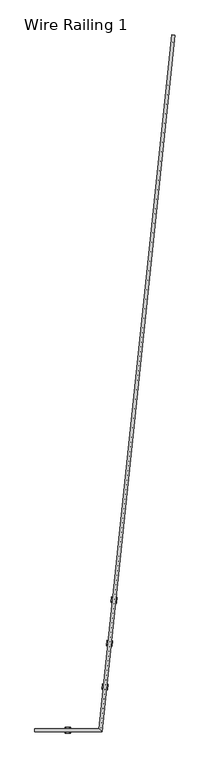
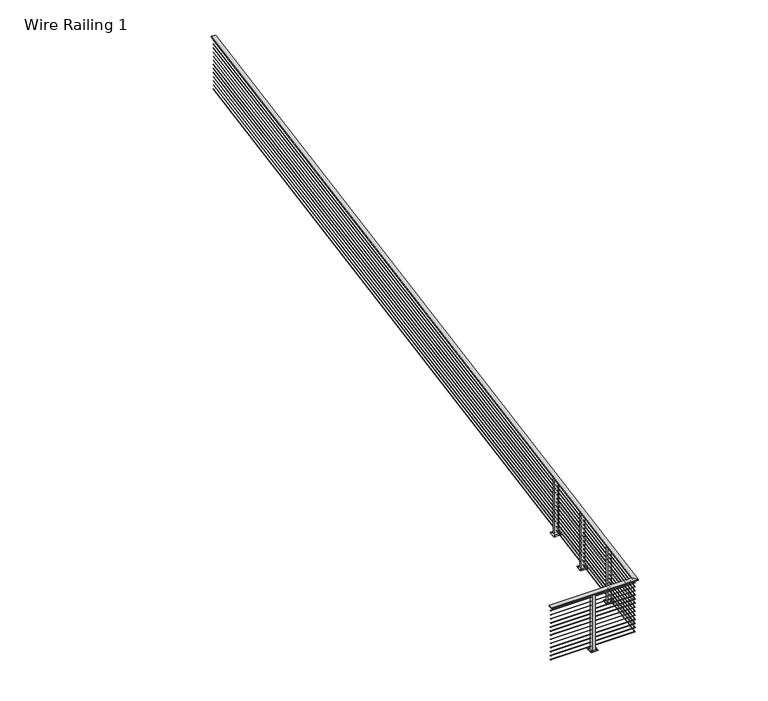
"""IFC4 building model written with IfcOpenShell, lengths in millimetres: railing geometry, Wire Railing 1."""

from ifc_helpers import new_model, si_unit, point, frame, frame_2d, origin, place, context, project, spatial, polyline, circle_curve, ellipse_curve, trimmed, segment, composite_curve, outline, extrude, faceted_brep, source, transform, mapped, element, save
from ifc_brep_helpers import plane_surface, cylinder_surface, advanced_brep


def wire_railing_1_8b9fc924(model_context):
    return source(origin(), model_context, "Body", "SolidModel", [
        faceted_brep([(32234.7381966, 25546.7031612, 267462.0), (32234.7381966, 25622.9031612, 267462.0), (32234.7381966, 25622.9031612, 267442.95), (32234.7381966, 25546.7031612, 267442.95), (33761.2935907, 25546.7031612, 267462.0), (33692.6828025, 25622.9031612, 267462.0), (33692.6828025, 25622.9031612, 267442.95), (33761.2935907, 25546.7031612, 267442.95), (35422.3408934, 41350.5125752, 267462.0), (35422.3408934, 41350.5125752, 267442.95), (35346.558325, 41358.4776441, 267442.95), (35346.558325, 41358.4776441, 267462.0)], [[[0, 1, 2, 3]], [[4, 5, 1, 0]], [[5, 6, 2, 1]], [[6, 7, 3, 2]], [[7, 4, 0, 3]], [[8, 9, 10, 11]], [[9, 8, 4, 7]], [[10, 9, 7, 6]], [[11, 10, 6, 5]], [[8, 11, 5, 4]]]),
        advanced_brep(
        [(32234.7381966, 25587.1844112, 267383.41875), (32234.7381966, 25582.4219112, 267383.41875), (33724.8441095, 25587.1844112, 267383.41875), (33729.1322837, 25582.4219112, 267383.41875), (35382.081404, 41354.7440181, 267383.41875), (35386.8178145, 41354.2462013, 267383.41875)],
        [
            (0, 1, circle_curve(frame((32234.7381966, 25584.8031612, 267383.41875), z_axis=(-1.0, 0.0, 0.0), x_axis=(0.0, -1.0, 0.0)), 2.38125)),
            (1, 0, circle_curve(frame((32234.7381966, 25584.8031612, 267383.41875), z_axis=(-1.0, 0.0, 0.0), x_axis=(0.0, -1.0, 0.0)), 2.38125)),
            (2, 3, ellipse_curve(frame((33726.9881966, 25584.8031612, 267383.41875), z_axis=(-0.7431448254773928, -0.66913060635886, 0.0), x_axis=(0.6691306063588597, -0.7431448254773928, 0.0)), 3.2042879, 2.38125)),
            (3, 1),
            (0, 2),
            (3, 2, ellipse_curve(frame((33726.9881966, 25584.8031612, 267383.41875), z_axis=(-0.7431448254773928, -0.66913060635886, 0.0), x_axis=(0.6691306063588597, -0.7431448254773928, 0.0)), 3.2042879, 2.38125)),
            (4, 5, circle_curve(frame((35384.4496092, 41354.4951097, 267383.41875), z_axis=(0.10452846326764917, 0.9945218953682738, 0.0), x_axis=(0.9945218953682738, -0.10452846326764917, 0.0)), 2.38125)),
            (5, 4, circle_curve(frame((35384.4496092, 41354.4951097, 267383.41875), z_axis=(0.10452846326764917, 0.9945218953682738, 0.0), x_axis=(0.9945218953682738, -0.10452846326764917, 0.0)), 2.38125)),
            (4, 2),
            (3, 5),
        ],
        [
            plane_surface(frame((32234.7381966, 25584.8031612, 267385.8), z_axis=(-1.0, 0.0, 0.0), x_axis=(0.0, -1.0, 0.0))),
            cylinder_surface(frame((33726.9881966, 25584.8031612, 267383.41875), z_axis=(1.0, 0.0, 0.0), x_axis=(0.0, -1.0, 0.0)), 2.38125),
            plane_surface(frame((35384.4496092, 41354.4951097, 267385.8), z_axis=(0.10452846326764917, 0.9945218953682738, 0.0), x_axis=(0.9945218953682738, -0.10452846326764917, 0.0))),
            cylinder_surface(frame((35384.4496092, 41354.4951097, 267383.41875), z_axis=(0.10452846326764917, 0.9945218953682738, 0.0), x_axis=(0.9945218953682738, -0.10452846326764917, 0.0)), 2.38125),
        ],
        [
            (0, [[1, 2]]),
            (1, [[3, 4, -1, 5]]),
            (1, [[6, -5, -2, -4]]),
            (2, [[7, 8]]),
            (3, [[-7, 9, -6, 10]]),
            (3, [[-8, -10, -3, -9]]),
        ],
    ),
        advanced_brep(
        [(32234.7381966, 25587.1844112, 267307.21875), (32234.7381966, 25582.4219112, 267307.21875), (33724.8441095, 25587.1844112, 267307.21875), (33729.1322837, 25582.4219112, 267307.21875), (35382.081404, 41354.7440181, 267307.21875), (35386.8178145, 41354.2462013, 267307.21875)],
        [
            (0, 1, circle_curve(frame((32234.7381966, 25584.8031612, 267307.21875), z_axis=(-1.0, 0.0, 0.0), x_axis=(0.0, -1.0, 0.0)), 2.38125)),
            (1, 0, circle_curve(frame((32234.7381966, 25584.8031612, 267307.21875), z_axis=(-1.0, 0.0, 0.0), x_axis=(0.0, -1.0, 0.0)), 2.38125)),
            (2, 3, ellipse_curve(frame((33726.9881966, 25584.8031612, 267307.21875), z_axis=(-0.7431448254773928, -0.66913060635886, 0.0), x_axis=(0.6691306063588597, -0.7431448254773928, 0.0)), 3.2042879, 2.38125)),
            (3, 1),
            (0, 2),
            (3, 2, ellipse_curve(frame((33726.9881966, 25584.8031612, 267307.21875), z_axis=(-0.7431448254773928, -0.66913060635886, 0.0), x_axis=(0.6691306063588597, -0.7431448254773928, 0.0)), 3.2042879, 2.38125)),
            (4, 5, circle_curve(frame((35384.4496092, 41354.4951097, 267307.21875), z_axis=(0.10452846326764917, 0.9945218953682738, 0.0), x_axis=(0.9945218953682738, -0.10452846326764917, 0.0)), 2.38125)),
            (5, 4, circle_curve(frame((35384.4496092, 41354.4951097, 267307.21875), z_axis=(0.10452846326764917, 0.9945218953682738, 0.0), x_axis=(0.9945218953682738, -0.10452846326764917, 0.0)), 2.38125)),
            (4, 2),
            (3, 5),
        ],
        [
            plane_surface(frame((32234.7381966, 25584.8031612, 267309.6), z_axis=(-1.0, 0.0, 0.0), x_axis=(0.0, -1.0, 0.0))),
            cylinder_surface(frame((33726.9881966, 25584.8031612, 267307.21875), z_axis=(1.0, 0.0, 0.0), x_axis=(0.0, -1.0, 0.0)), 2.38125),
            plane_surface(frame((35384.4496092, 41354.4951097, 267309.6), z_axis=(0.10452846326764917, 0.9945218953682738, 0.0), x_axis=(0.9945218953682738, -0.10452846326764917, 0.0))),
            cylinder_surface(frame((35384.4496092, 41354.4951097, 267307.21875), z_axis=(0.10452846326764917, 0.9945218953682738, 0.0), x_axis=(0.9945218953682738, -0.10452846326764917, 0.0)), 2.38125),
        ],
        [
            (0, [[1, 2]]),
            (1, [[3, 4, -1, 5]]),
            (1, [[6, -5, -2, -4]]),
            (2, [[7, 8]]),
            (3, [[-7, 9, -6, 10]]),
            (3, [[-8, -10, -3, -9]]),
        ],
    ),
        advanced_brep(
        [(32234.7381966, 25587.1844112, 267231.01875), (32234.7381966, 25582.4219112, 267231.01875), (33724.8441095, 25587.1844112, 267231.01875), (33729.1322837, 25582.4219112, 267231.01875), (35382.081404, 41354.7440181, 267231.01875), (35386.8178145, 41354.2462013, 267231.01875)],
        [
            (0, 1, circle_curve(frame((32234.7381966, 25584.8031612, 267231.01875), z_axis=(-1.0, 0.0, 0.0), x_axis=(0.0, -1.0, 0.0)), 2.38125)),
            (1, 0, circle_curve(frame((32234.7381966, 25584.8031612, 267231.01875), z_axis=(-1.0, 0.0, 0.0), x_axis=(0.0, -1.0, 0.0)), 2.38125)),
            (2, 3, ellipse_curve(frame((33726.9881966, 25584.8031612, 267231.01875), z_axis=(-0.7431448254773928, -0.66913060635886, 0.0), x_axis=(0.6691306063588597, -0.7431448254773928, 0.0)), 3.2042879, 2.38125)),
            (3, 1),
            (0, 2),
            (3, 2, ellipse_curve(frame((33726.9881966, 25584.8031612, 267231.01875), z_axis=(-0.7431448254773928, -0.66913060635886, 0.0), x_axis=(0.6691306063588597, -0.7431448254773928, 0.0)), 3.2042879, 2.38125)),
            (4, 5, circle_curve(frame((35384.4496092, 41354.4951097, 267231.01875), z_axis=(0.10452846326764917, 0.9945218953682738, 0.0), x_axis=(0.9945218953682738, -0.10452846326764917, 0.0)), 2.38125)),
            (5, 4, circle_curve(frame((35384.4496092, 41354.4951097, 267231.01875), z_axis=(0.10452846326764917, 0.9945218953682738, 0.0), x_axis=(0.9945218953682738, -0.10452846326764917, 0.0)), 2.38125)),
            (4, 2),
            (3, 5),
        ],
        [
            plane_surface(frame((32234.7381966, 25584.8031612, 267233.4), z_axis=(-1.0, 0.0, 0.0), x_axis=(0.0, -1.0, 0.0))),
            cylinder_surface(frame((33726.9881966, 25584.8031612, 267231.01875), z_axis=(1.0, 0.0, 0.0), x_axis=(0.0, -1.0, 0.0)), 2.38125),
            plane_surface(frame((35384.4496092, 41354.4951097, 267233.4), z_axis=(0.10452846326764917, 0.9945218953682738, 0.0), x_axis=(0.9945218953682738, -0.10452846326764917, 0.0))),
            cylinder_surface(frame((35384.4496092, 41354.4951097, 267231.01875), z_axis=(0.10452846326764917, 0.9945218953682738, 0.0), x_axis=(0.9945218953682738, -0.10452846326764917, 0.0)), 2.38125),
        ],
        [
            (0, [[1, 2]]),
            (1, [[3, 4, -1, 5]]),
            (1, [[6, -5, -2, -4]]),
            (2, [[7, 8]]),
            (3, [[-7, 9, -6, 10]]),
            (3, [[-8, -10, -3, -9]]),
        ],
    ),
        advanced_brep(
        [(32234.7381966, 25587.1844112, 267154.81875), (32234.7381966, 25582.4219112, 267154.81875), (33724.8441095, 25587.1844112, 267154.81875), (33729.1322837, 25582.4219112, 267154.81875), (35382.081404, 41354.7440181, 267154.81875), (35386.8178145, 41354.2462013, 267154.81875)],
        [
            (0, 1, circle_curve(frame((32234.7381966, 25584.8031612, 267154.81875), z_axis=(-1.0, 0.0, 0.0), x_axis=(0.0, -1.0, 0.0)), 2.38125)),
            (1, 0, circle_curve(frame((32234.7381966, 25584.8031612, 267154.81875), z_axis=(-1.0, 0.0, 0.0), x_axis=(0.0, -1.0, 0.0)), 2.38125)),
            (2, 3, ellipse_curve(frame((33726.9881966, 25584.8031612, 267154.81875), z_axis=(-0.7431448254773928, -0.66913060635886, 0.0), x_axis=(0.6691306063588597, -0.7431448254773928, 0.0)), 3.2042879, 2.38125)),
            (3, 1),
            (0, 2),
            (3, 2, ellipse_curve(frame((33726.9881966, 25584.8031612, 267154.81875), z_axis=(-0.7431448254773928, -0.66913060635886, 0.0), x_axis=(0.6691306063588597, -0.7431448254773928, 0.0)), 3.2042879, 2.38125)),
            (4, 5, circle_curve(frame((35384.4496092, 41354.4951097, 267154.81875), z_axis=(0.10452846326764917, 0.9945218953682738, 0.0), x_axis=(0.9945218953682738, -0.10452846326764917, 0.0)), 2.38125)),
            (5, 4, circle_curve(frame((35384.4496092, 41354.4951097, 267154.81875), z_axis=(0.10452846326764917, 0.9945218953682738, 0.0), x_axis=(0.9945218953682738, -0.10452846326764917, 0.0)), 2.38125)),
            (4, 2),
            (3, 5),
        ],
        [
            plane_surface(frame((32234.7381966, 25584.8031612, 267157.2), z_axis=(-1.0, 0.0, 0.0), x_axis=(0.0, -1.0, 0.0))),
            cylinder_surface(frame((33726.9881966, 25584.8031612, 267154.81875), z_axis=(1.0, 0.0, 0.0), x_axis=(0.0, -1.0, 0.0)), 2.38125),
            plane_surface(frame((35384.4496092, 41354.4951097, 267157.2), z_axis=(0.10452846326764917, 0.9945218953682738, 0.0), x_axis=(0.9945218953682738, -0.10452846326764917, 0.0))),
            cylinder_surface(frame((35384.4496092, 41354.4951097, 267154.81875), z_axis=(0.10452846326764917, 0.9945218953682738, 0.0), x_axis=(0.9945218953682738, -0.10452846326764917, 0.0)), 2.38125),
        ],
        [
            (0, [[1, 2]]),
            (1, [[3, 4, -1, 5]]),
            (1, [[6, -5, -2, -4]]),
            (2, [[7, 8]]),
            (3, [[-7, 9, -6, 10]]),
            (3, [[-8, -10, -3, -9]]),
        ],
    ),
        advanced_brep(
        [(32234.7381966, 25587.1844112, 267078.61875), (32234.7381966, 25582.4219112, 267078.61875), (33724.8441095, 25587.1844112, 267078.61875), (33729.1322837, 25582.4219112, 267078.61875), (35382.081404, 41354.7440181, 267078.61875), (35386.8178145, 41354.2462013, 267078.61875)],
        [
            (0, 1, circle_curve(frame((32234.7381966, 25584.8031612, 267078.61875), z_axis=(-1.0, 0.0, 0.0), x_axis=(0.0, -1.0, 0.0)), 2.38125)),
            (1, 0, circle_curve(frame((32234.7381966, 25584.8031612, 267078.61875), z_axis=(-1.0, 0.0, 0.0), x_axis=(0.0, -1.0, 0.0)), 2.38125)),
            (2, 3, ellipse_curve(frame((33726.9881966, 25584.8031612, 267078.61875), z_axis=(-0.7431448254773928, -0.66913060635886, 0.0), x_axis=(0.6691306063588597, -0.7431448254773928, 0.0)), 3.2042879, 2.38125)),
            (3, 1),
            (0, 2),
            (3, 2, ellipse_curve(frame((33726.9881966, 25584.8031612, 267078.61875), z_axis=(-0.7431448254773928, -0.66913060635886, 0.0), x_axis=(0.6691306063588597, -0.7431448254773928, 0.0)), 3.2042879, 2.38125)),
            (4, 5, circle_curve(frame((35384.4496092, 41354.4951097, 267078.61875), z_axis=(0.10452846326764917, 0.9945218953682738, 0.0), x_axis=(0.9945218953682738, -0.10452846326764917, 0.0)), 2.38125)),
            (5, 4, circle_curve(frame((35384.4496092, 41354.4951097, 267078.61875), z_axis=(0.10452846326764917, 0.9945218953682738, 0.0), x_axis=(0.9945218953682738, -0.10452846326764917, 0.0)), 2.38125)),
            (4, 2),
            (3, 5),
        ],
        [
            plane_surface(frame((32234.7381966, 25584.8031612, 267081.0), z_axis=(-1.0, 0.0, 0.0), x_axis=(0.0, -1.0, 0.0))),
            cylinder_surface(frame((33726.9881966, 25584.8031612, 267078.61875), z_axis=(1.0, 0.0, 0.0), x_axis=(0.0, -1.0, 0.0)), 2.38125),
            plane_surface(frame((35384.4496092, 41354.4951097, 267081.0), z_axis=(0.10452846326764917, 0.9945218953682738, 0.0), x_axis=(0.9945218953682738, -0.10452846326764917, 0.0))),
            cylinder_surface(frame((35384.4496092, 41354.4951097, 267078.61875), z_axis=(0.10452846326764917, 0.9945218953682738, 0.0), x_axis=(0.9945218953682738, -0.10452846326764917, 0.0)), 2.38125),
        ],
        [
            (0, [[1, 2]]),
            (1, [[3, 4, -1, 5]]),
            (1, [[6, -5, -2, -4]]),
            (2, [[7, 8]]),
            (3, [[-7, 9, -6, 10]]),
            (3, [[-8, -10, -3, -9]]),
        ],
    ),
        advanced_brep(
        [(32234.7381966, 25587.1844112, 267002.41875), (32234.7381966, 25582.4219112, 267002.41875), (33724.8441095, 25587.1844112, 267002.41875), (33729.1322837, 25582.4219112, 267002.41875), (35382.081404, 41354.7440181, 267002.41875), (35386.8178145, 41354.2462013, 267002.41875)],
        [
            (0, 1, circle_curve(frame((32234.7381966, 25584.8031612, 267002.41875), z_axis=(-1.0, 0.0, 0.0), x_axis=(0.0, -1.0, 0.0)), 2.38125)),
            (1, 0, circle_curve(frame((32234.7381966, 25584.8031612, 267002.41875), z_axis=(-1.0, 0.0, 0.0), x_axis=(0.0, -1.0, 0.0)), 2.38125)),
            (2, 3, ellipse_curve(frame((33726.9881966, 25584.8031612, 267002.41875), z_axis=(-0.7431448254773928, -0.66913060635886, 0.0), x_axis=(0.6691306063588597, -0.7431448254773928, 0.0)), 3.2042879, 2.38125)),
            (3, 1),
            (0, 2),
            (3, 2, ellipse_curve(frame((33726.9881966, 25584.8031612, 267002.41875), z_axis=(-0.7431448254773928, -0.66913060635886, 0.0), x_axis=(0.6691306063588597, -0.7431448254773928, 0.0)), 3.2042879, 2.38125)),
            (4, 5, circle_curve(frame((35384.4496092, 41354.4951097, 267002.41875), z_axis=(0.10452846326764917, 0.9945218953682738, 0.0), x_axis=(0.9945218953682738, -0.10452846326764917, 0.0)), 2.38125)),
            (5, 4, circle_curve(frame((35384.4496092, 41354.4951097, 267002.41875), z_axis=(0.10452846326764917, 0.9945218953682738, 0.0), x_axis=(0.9945218953682738, -0.10452846326764917, 0.0)), 2.38125)),
            (4, 2),
            (3, 5),
        ],
        [
            plane_surface(frame((32234.7381966, 25584.8031612, 267004.8), z_axis=(-1.0, 0.0, 0.0), x_axis=(0.0, -1.0, 0.0))),
            cylinder_surface(frame((33726.9881966, 25584.8031612, 267002.41875), z_axis=(1.0, 0.0, 0.0), x_axis=(0.0, -1.0, 0.0)), 2.38125),
            plane_surface(frame((35384.4496092, 41354.4951097, 267004.8), z_axis=(0.10452846326764917, 0.9945218953682738, 0.0), x_axis=(0.9945218953682738, -0.10452846326764917, 0.0))),
            cylinder_surface(frame((35384.4496092, 41354.4951097, 267002.41875), z_axis=(0.10452846326764917, 0.9945218953682738, 0.0), x_axis=(0.9945218953682738, -0.10452846326764917, 0.0)), 2.38125),
        ],
        [
            (0, [[1, 2]]),
            (1, [[3, 4, -1, 5]]),
            (1, [[6, -5, -2, -4]]),
            (2, [[7, 8]]),
            (3, [[-7, 9, -6, 10]]),
            (3, [[-8, -10, -3, -9]]),
        ],
    ),
        advanced_brep(
        [(32234.7381966, 25587.1844112, 266926.21875), (32234.7381966, 25582.4219112, 266926.21875), (33724.8441095, 25587.1844112, 266926.21875), (33729.1322837, 25582.4219112, 266926.21875), (35382.081404, 41354.7440181, 266926.21875), (35386.8178145, 41354.2462013, 266926.21875)],
        [
            (0, 1, circle_curve(frame((32234.7381966, 25584.8031612, 266926.21875), z_axis=(-1.0, 0.0, 0.0), x_axis=(0.0, -1.0, 0.0)), 2.38125)),
            (1, 0, circle_curve(frame((32234.7381966, 25584.8031612, 266926.21875), z_axis=(-1.0, 0.0, 0.0), x_axis=(0.0, -1.0, 0.0)), 2.38125)),
            (2, 3, ellipse_curve(frame((33726.9881966, 25584.8031612, 266926.21875), z_axis=(-0.7431448254773928, -0.66913060635886, 0.0), x_axis=(0.6691306063588597, -0.7431448254773928, 0.0)), 3.2042879, 2.38125)),
            (3, 1),
            (0, 2),
            (3, 2, ellipse_curve(frame((33726.9881966, 25584.8031612, 266926.21875), z_axis=(-0.7431448254773928, -0.66913060635886, 0.0), x_axis=(0.6691306063588597, -0.7431448254773928, 0.0)), 3.2042879, 2.38125)),
            (4, 5, circle_curve(frame((35384.4496092, 41354.4951097, 266926.21875), z_axis=(0.10452846326764917, 0.9945218953682738, 0.0), x_axis=(0.9945218953682738, -0.10452846326764917, 0.0)), 2.38125)),
            (5, 4, circle_curve(frame((35384.4496092, 41354.4951097, 266926.21875), z_axis=(0.10452846326764917, 0.9945218953682738, 0.0), x_axis=(0.9945218953682738, -0.10452846326764917, 0.0)), 2.38125)),
            (4, 2),
            (3, 5),
        ],
        [
            plane_surface(frame((32234.7381966, 25584.8031612, 266928.6), z_axis=(-1.0, 0.0, 0.0), x_axis=(0.0, -1.0, 0.0))),
            cylinder_surface(frame((33726.9881966, 25584.8031612, 266926.21875), z_axis=(1.0, 0.0, 0.0), x_axis=(0.0, -1.0, 0.0)), 2.38125),
            plane_surface(frame((35384.4496092, 41354.4951097, 266928.6), z_axis=(0.10452846326764917, 0.9945218953682738, 0.0), x_axis=(0.9945218953682738, -0.10452846326764917, 0.0))),
            cylinder_surface(frame((35384.4496092, 41354.4951097, 266926.21875), z_axis=(0.10452846326764917, 0.9945218953682738, 0.0), x_axis=(0.9945218953682738, -0.10452846326764917, 0.0)), 2.38125),
        ],
        [
            (0, [[1, 2]]),
            (1, [[3, 4, -1, 5]]),
            (1, [[6, -5, -2, -4]]),
            (2, [[7, 8]]),
            (3, [[-7, 9, -6, 10]]),
            (3, [[-8, -10, -3, -9]]),
        ],
    ),
        advanced_brep(
        [(32234.7381966, 25587.1844112, 266850.01875), (32234.7381966, 25582.4219112, 266850.01875), (33724.8441095, 25587.1844112, 266850.01875), (33729.1322837, 25582.4219112, 266850.01875), (35382.081404, 41354.7440181, 266850.01875), (35386.8178145, 41354.2462013, 266850.01875)],
        [
            (0, 1, circle_curve(frame((32234.7381966, 25584.8031612, 266850.01875), z_axis=(-1.0, 0.0, 0.0), x_axis=(0.0, -1.0, 0.0)), 2.38125)),
            (1, 0, circle_curve(frame((32234.7381966, 25584.8031612, 266850.01875), z_axis=(-1.0, 0.0, 0.0), x_axis=(0.0, -1.0, 0.0)), 2.38125)),
            (2, 3, ellipse_curve(frame((33726.9881966, 25584.8031612, 266850.01875), z_axis=(-0.7431448254773928, -0.66913060635886, 0.0), x_axis=(0.6691306063588597, -0.7431448254773928, 0.0)), 3.2042879, 2.38125)),
            (3, 1),
            (0, 2),
            (3, 2, ellipse_curve(frame((33726.9881966, 25584.8031612, 266850.01875), z_axis=(-0.7431448254773928, -0.66913060635886, 0.0), x_axis=(0.6691306063588597, -0.7431448254773928, 0.0)), 3.2042879, 2.38125)),
            (4, 5, circle_curve(frame((35384.4496092, 41354.4951097, 266850.01875), z_axis=(0.10452846326764917, 0.9945218953682738, 0.0), x_axis=(0.9945218953682738, -0.10452846326764917, 0.0)), 2.38125)),
            (5, 4, circle_curve(frame((35384.4496092, 41354.4951097, 266850.01875), z_axis=(0.10452846326764917, 0.9945218953682738, 0.0), x_axis=(0.9945218953682738, -0.10452846326764917, 0.0)), 2.38125)),
            (4, 2),
            (3, 5),
        ],
        [
            plane_surface(frame((32234.7381966, 25584.8031612, 266852.4), z_axis=(-1.0, 0.0, 0.0), x_axis=(0.0, -1.0, 0.0))),
            cylinder_surface(frame((33726.9881966, 25584.8031612, 266850.01875), z_axis=(1.0, 0.0, 0.0), x_axis=(0.0, -1.0, 0.0)), 2.38125),
            plane_surface(frame((35384.4496092, 41354.4951097, 266852.4), z_axis=(0.10452846326764917, 0.9945218953682738, 0.0), x_axis=(0.9945218953682738, -0.10452846326764917, 0.0))),
            cylinder_surface(frame((35384.4496092, 41354.4951097, 266850.01875), z_axis=(0.10452846326764917, 0.9945218953682738, 0.0), x_axis=(0.9945218953682738, -0.10452846326764917, 0.0)), 2.38125),
        ],
        [
            (0, [[1, 2]]),
            (1, [[3, 4, -1, 5]]),
            (1, [[6, -5, -2, -4]]),
            (2, [[7, 8]]),
            (3, [[-7, 9, -6, 10]]),
            (3, [[-8, -10, -3, -9]]),
        ],
    ),
        advanced_brep(
        [(32234.7381966, 25587.1844112, 266773.81875), (32234.7381966, 25582.4219112, 266773.81875), (33724.8441095, 25587.1844112, 266773.81875), (33729.1322837, 25582.4219112, 266773.81875), (35382.081404, 41354.7440181, 266773.81875), (35386.8178145, 41354.2462013, 266773.81875)],
        [
            (0, 1, circle_curve(frame((32234.7381966, 25584.8031612, 266773.81875), z_axis=(-1.0, 0.0, 0.0), x_axis=(0.0, -1.0, 0.0)), 2.38125)),
            (1, 0, circle_curve(frame((32234.7381966, 25584.8031612, 266773.81875), z_axis=(-1.0, 0.0, 0.0), x_axis=(0.0, -1.0, 0.0)), 2.38125)),
            (2, 3, ellipse_curve(frame((33726.9881966, 25584.8031612, 266773.81875), z_axis=(-0.7431448254773928, -0.66913060635886, 0.0), x_axis=(0.6691306063588597, -0.7431448254773928, 0.0)), 3.2042879, 2.38125)),
            (3, 1),
            (0, 2),
            (3, 2, ellipse_curve(frame((33726.9881966, 25584.8031612, 266773.81875), z_axis=(-0.7431448254773928, -0.66913060635886, 0.0), x_axis=(0.6691306063588597, -0.7431448254773928, 0.0)), 3.2042879, 2.38125)),
            (4, 5, circle_curve(frame((35384.4496092, 41354.4951097, 266773.81875), z_axis=(0.10452846326764917, 0.9945218953682738, 0.0), x_axis=(0.9945218953682738, -0.10452846326764917, 0.0)), 2.38125)),
            (5, 4, circle_curve(frame((35384.4496092, 41354.4951097, 266773.81875), z_axis=(0.10452846326764917, 0.9945218953682738, 0.0), x_axis=(0.9945218953682738, -0.10452846326764917, 0.0)), 2.38125)),
            (4, 2),
            (3, 5),
        ],
        [
            plane_surface(frame((32234.7381966, 25584.8031612, 266776.2), z_axis=(-1.0, 0.0, 0.0), x_axis=(0.0, -1.0, 0.0))),
            cylinder_surface(frame((33726.9881966, 25584.8031612, 266773.81875), z_axis=(1.0, 0.0, 0.0), x_axis=(0.0, -1.0, 0.0)), 2.38125),
            plane_surface(frame((35384.4496092, 41354.4951097, 266776.2), z_axis=(0.10452846326764917, 0.9945218953682738, 0.0), x_axis=(0.9945218953682738, -0.10452846326764917, 0.0))),
            cylinder_surface(frame((35384.4496092, 41354.4951097, 266773.81875), z_axis=(0.10452846326764917, 0.9945218953682738, 0.0), x_axis=(0.9945218953682738, -0.10452846326764917, 0.0)), 2.38125),
        ],
        [
            (0, [[1, 2]]),
            (1, [[3, 4, -1, 5]]),
            (1, [[6, -5, -2, -4]]),
            (2, [[7, 8]]),
            (3, [[-7, 9, -6, 10]]),
            (3, [[-8, -10, -3, -9]]),
        ],
    ),
        advanced_brep(
        [(32234.7381966, 25587.1844112, 266697.61875), (32234.7381966, 25582.4219112, 266697.61875), (33724.8441095, 25587.1844112, 266697.61875), (33729.1322837, 25582.4219112, 266697.61875), (35382.081404, 41354.7440181, 266697.61875), (35386.8178145, 41354.2462013, 266697.61875)],
        [
            (0, 1, circle_curve(frame((32234.7381966, 25584.8031612, 266697.61875), z_axis=(-1.0, 0.0, 0.0), x_axis=(0.0, -1.0, 0.0)), 2.38125)),
            (1, 0, circle_curve(frame((32234.7381966, 25584.8031612, 266697.61875), z_axis=(-1.0, 0.0, 0.0), x_axis=(0.0, -1.0, 0.0)), 2.38125)),
            (2, 3, ellipse_curve(frame((33726.9881966, 25584.8031612, 266697.61875), z_axis=(-0.7431448254773928, -0.66913060635886, 0.0), x_axis=(0.6691306063588597, -0.7431448254773928, 0.0)), 3.2042879, 2.38125)),
            (3, 1),
            (0, 2),
            (3, 2, ellipse_curve(frame((33726.9881966, 25584.8031612, 266697.61875), z_axis=(-0.7431448254773928, -0.66913060635886, 0.0), x_axis=(0.6691306063588597, -0.7431448254773928, 0.0)), 3.2042879, 2.38125)),
            (4, 5, circle_curve(frame((35384.4496092, 41354.4951097, 266697.61875), z_axis=(0.10452846326764917, 0.9945218953682738, 0.0), x_axis=(0.9945218953682738, -0.10452846326764917, 0.0)), 2.38125)),
            (5, 4, circle_curve(frame((35384.4496092, 41354.4951097, 266697.61875), z_axis=(0.10452846326764917, 0.9945218953682738, 0.0), x_axis=(0.9945218953682738, -0.10452846326764917, 0.0)), 2.38125)),
            (4, 2),
            (3, 5),
        ],
        [
            plane_surface(frame((32234.7381966, 25584.8031612, 266700.0), z_axis=(-1.0, 0.0, 0.0), x_axis=(0.0, -1.0, 0.0))),
            cylinder_surface(frame((33726.9881966, 25584.8031612, 266697.61875), z_axis=(1.0, 0.0, 0.0), x_axis=(0.0, -1.0, 0.0)), 2.38125),
            plane_surface(frame((35384.4496092, 41354.4951097, 266700.0), z_axis=(0.10452846326764917, 0.9945218953682738, 0.0), x_axis=(0.9945218953682738, -0.10452846326764917, 0.0))),
            cylinder_surface(frame((35384.4496092, 41354.4951097, 266697.61875), z_axis=(0.10452846326764917, 0.9945218953682738, 0.0), x_axis=(0.9945218953682738, -0.10452846326764917, 0.0)), 2.38125),
        ],
        [
            (0, [[1, 2]]),
            (1, [[3, 4, -1, 5]]),
            (1, [[6, -5, -2, -4]]),
            (2, [[7, 8]]),
            (3, [[-7, 9, -6, 10]]),
            (3, [[-8, -10, -3, -9]]),
        ],
    ),
        advanced_brep(
        [(32234.7381966, 25587.1844112, 266621.41875), (32234.7381966, 25582.4219112, 266621.41875), (33724.8441095, 25587.1844112, 266621.41875), (33729.1322837, 25582.4219112, 266621.41875), (35382.081404, 41354.7440181, 266621.41875), (35386.8178145, 41354.2462013, 266621.41875)],
        [
            (0, 1, circle_curve(frame((32234.7381966, 25584.8031612, 266621.41875), z_axis=(-1.0, 0.0, 0.0), x_axis=(0.0, -1.0, 0.0)), 2.38125)),
            (1, 0, circle_curve(frame((32234.7381966, 25584.8031612, 266621.41875), z_axis=(-1.0, 0.0, 0.0), x_axis=(0.0, -1.0, 0.0)), 2.38125)),
            (2, 3, ellipse_curve(frame((33726.9881966, 25584.8031612, 266621.41875), z_axis=(-0.7431448254773928, -0.66913060635886, 0.0), x_axis=(0.6691306063588597, -0.7431448254773928, 0.0)), 3.2042879, 2.38125)),
            (3, 1),
            (0, 2),
            (3, 2, ellipse_curve(frame((33726.9881966, 25584.8031612, 266621.41875), z_axis=(-0.7431448254773928, -0.66913060635886, 0.0), x_axis=(0.6691306063588597, -0.7431448254773928, 0.0)), 3.2042879, 2.38125)),
            (4, 5, circle_curve(frame((35384.4496092, 41354.4951097, 266621.41875), z_axis=(0.10452846326764917, 0.9945218953682738, 0.0), x_axis=(0.9945218953682738, -0.10452846326764917, 0.0)), 2.38125)),
            (5, 4, circle_curve(frame((35384.4496092, 41354.4951097, 266621.41875), z_axis=(0.10452846326764917, 0.9945218953682738, 0.0), x_axis=(0.9945218953682738, -0.10452846326764917, 0.0)), 2.38125)),
            (4, 2),
            (3, 5),
        ],
        [
            plane_surface(frame((32234.7381966, 25584.8031612, 266623.8), z_axis=(-1.0, 0.0, 0.0), x_axis=(0.0, -1.0, 0.0))),
            cylinder_surface(frame((33726.9881966, 25584.8031612, 266621.41875), z_axis=(1.0, 0.0, 0.0), x_axis=(0.0, -1.0, 0.0)), 2.38125),
            plane_surface(frame((35384.4496092, 41354.4951097, 266623.8), z_axis=(0.10452846326764917, 0.9945218953682738, 0.0), x_axis=(0.9945218953682738, -0.10452846326764917, 0.0))),
            cylinder_surface(frame((35384.4496092, 41354.4951097, 266621.41875), z_axis=(0.10452846326764917, 0.9945218953682738, 0.0), x_axis=(0.9945218953682738, -0.10452846326764917, 0.0)), 2.38125),
        ],
        [
            (0, [[1, 2]]),
            (1, [[3, 4, -1, 5]]),
            (1, [[6, -5, -2, -4]]),
            (2, [[7, 8]]),
            (3, [[-7, 9, -6, 10]]),
            (3, [[-8, -10, -3, -9]]),
        ],
    ),
        advanced_brep(
        [(32234.7381966, 25587.1844112, 266545.21875), (32234.7381966, 25582.4219112, 266545.21875), (33724.8441095, 25587.1844112, 266545.21875), (33729.1322837, 25582.4219112, 266545.21875), (35382.081404, 41354.7440181, 266545.21875), (35386.8178145, 41354.2462013, 266545.21875)],
        [
            (0, 1, circle_curve(frame((32234.7381966, 25584.8031612, 266545.21875), z_axis=(-1.0, 0.0, 0.0), x_axis=(0.0, -1.0, 0.0)), 2.38125)),
            (1, 0, circle_curve(frame((32234.7381966, 25584.8031612, 266545.21875), z_axis=(-1.0, 0.0, 0.0), x_axis=(0.0, -1.0, 0.0)), 2.38125)),
            (2, 3, ellipse_curve(frame((33726.9881966, 25584.8031612, 266545.21875), z_axis=(-0.7431448254773928, -0.66913060635886, 0.0), x_axis=(0.6691306063588597, -0.7431448254773928, 0.0)), 3.2042879, 2.38125)),
            (3, 1),
            (0, 2),
            (3, 2, ellipse_curve(frame((33726.9881966, 25584.8031612, 266545.21875), z_axis=(-0.7431448254773928, -0.66913060635886, 0.0), x_axis=(0.6691306063588597, -0.7431448254773928, 0.0)), 3.2042879, 2.38125)),
            (4, 5, circle_curve(frame((35384.4496092, 41354.4951097, 266545.21875), z_axis=(0.10452846326764917, 0.9945218953682738, 0.0), x_axis=(0.9945218953682738, -0.10452846326764917, 0.0)), 2.38125)),
            (5, 4, circle_curve(frame((35384.4496092, 41354.4951097, 266545.21875), z_axis=(0.10452846326764917, 0.9945218953682738, 0.0), x_axis=(0.9945218953682738, -0.10452846326764917, 0.0)), 2.38125)),
            (4, 2),
            (3, 5),
        ],
        [
            plane_surface(frame((32234.7381966, 25584.8031612, 266547.6), z_axis=(-1.0, 0.0, 0.0), x_axis=(0.0, -1.0, 0.0))),
            cylinder_surface(frame((33726.9881966, 25584.8031612, 266545.21875), z_axis=(1.0, 0.0, 0.0), x_axis=(0.0, -1.0, 0.0)), 2.38125),
            plane_surface(frame((35384.4496092, 41354.4951097, 266547.6), z_axis=(0.10452846326764917, 0.9945218953682738, 0.0), x_axis=(0.9945218953682738, -0.10452846326764917, 0.0))),
            cylinder_surface(frame((35384.4496092, 41354.4951097, 266545.21875), z_axis=(0.10452846326764917, 0.9945218953682738, 0.0), x_axis=(0.9945218953682738, -0.10452846326764917, 0.0)), 2.38125),
        ],
        [
            (0, [[1, 2]]),
            (1, [[3, 4, -1, 5]]),
            (1, [[6, -5, -2, -4]]),
            (2, [[7, 8]]),
            (3, [[-7, 9, -6, 10]]),
            (3, [[-8, -10, -3, -9]]),
        ],
    ),
        advanced_brep(
        [(32234.7381966, 25587.1844112, 266469.01875), (32234.7381966, 25582.4219112, 266469.01875), (33724.8441095, 25587.1844112, 266469.01875), (33729.1322837, 25582.4219112, 266469.01875), (35382.081404, 41354.7440181, 266469.01875), (35386.8178145, 41354.2462013, 266469.01875)],
        [
            (0, 1, circle_curve(frame((32234.7381966, 25584.8031612, 266469.01875), z_axis=(-1.0, 0.0, 0.0), x_axis=(0.0, -1.0, 0.0)), 2.38125)),
            (1, 0, circle_curve(frame((32234.7381966, 25584.8031612, 266469.01875), z_axis=(-1.0, 0.0, 0.0), x_axis=(0.0, -1.0, 0.0)), 2.38125)),
            (2, 3, ellipse_curve(frame((33726.9881966, 25584.8031612, 266469.01875), z_axis=(-0.7431448254773928, -0.66913060635886, 0.0), x_axis=(0.6691306063588597, -0.7431448254773928, 0.0)), 3.2042879, 2.38125)),
            (3, 1),
            (0, 2),
            (3, 2, ellipse_curve(frame((33726.9881966, 25584.8031612, 266469.01875), z_axis=(-0.7431448254773928, -0.66913060635886, 0.0), x_axis=(0.6691306063588597, -0.7431448254773928, 0.0)), 3.2042879, 2.38125)),
            (4, 5, circle_curve(frame((35384.4496092, 41354.4951097, 266469.01875), z_axis=(0.10452846326764917, 0.9945218953682738, 0.0), x_axis=(0.9945218953682738, -0.10452846326764917, 0.0)), 2.38125)),
            (5, 4, circle_curve(frame((35384.4496092, 41354.4951097, 266469.01875), z_axis=(0.10452846326764917, 0.9945218953682738, 0.0), x_axis=(0.9945218953682738, -0.10452846326764917, 0.0)), 2.38125)),
            (4, 2),
            (3, 5),
        ],
        [
            plane_surface(frame((32234.7381966, 25584.8031612, 266471.4), z_axis=(-1.0, 0.0, 0.0), x_axis=(0.0, -1.0, 0.0))),
            cylinder_surface(frame((33726.9881966, 25584.8031612, 266469.01875), z_axis=(1.0, 0.0, 0.0), x_axis=(0.0, -1.0, 0.0)), 2.38125),
            plane_surface(frame((35384.4496092, 41354.4951097, 266471.4), z_axis=(0.10452846326764917, 0.9945218953682738, 0.0), x_axis=(0.9945218953682738, -0.10452846326764917, 0.0))),
            cylinder_surface(frame((35384.4496092, 41354.4951097, 266469.01875), z_axis=(0.10452846326764917, 0.9945218953682738, 0.0), x_axis=(0.9945218953682738, -0.10452846326764917, 0.0)), 2.38125),
        ],
        [
            (0, [[1, 2]]),
            (1, [[3, 4, -1, 5]]),
            (1, [[6, -5, -2, -4]]),
            (2, [[7, 8]]),
            (3, [[-7, 9, -6, 10]]),
            (3, [[-8, -10, -3, -9]]),
        ],
    ),
        extrude(outline(composite_curve([segment(trimmed(circle_curve(frame_2d((33025.3131966, 25540.3531612)), 6.35), [point((33025.3131966, 25534.0031612))], [point((33025.3131966, 25546.7031612))], False, "CARTESIAN"), True, "CONTINUOUS"), segment(trimmed(circle_curve(frame_2d((33025.3131966, 25540.3531612)), 6.35), [point((33025.3131966, 25546.7031612))], [point((33025.3131966, 25534.0031612))], False, "CARTESIAN"), True, "CONTINUOUS")], self_intersect=False)), frame((0.0, 0.0, 266395.2), z_axis=(0.0, 0.0, 1.0), x_axis=(1.0, 0.0, 0.0)), (0.0, 0.0, 1.0), 12.7),
        extrude(outline(composite_curve([segment(trimmed(circle_curve(frame_2d((33025.3131966, 25629.2531612)), 6.35), [point((33025.3131966, 25622.9031612))], [point((33025.3131966, 25635.6031612))], False, "CARTESIAN"), True, "CONTINUOUS"), segment(trimmed(circle_curve(frame_2d((33025.3131966, 25629.2531612)), 6.35), [point((33025.3131966, 25635.6031612))], [point((33025.3131966, 25622.9031612))], False, "CARTESIAN"), True, "CONTINUOUS")], self_intersect=False)), frame((0.0, 0.0, 266395.2), z_axis=(0.0, 0.0, 1.0), x_axis=(1.0, 0.0, 0.0)), (0.0, 0.0, 1.0), 12.7),
        extrude(outline(composite_curve([segment(trimmed(circle_curve(frame_2d((32936.4131966, 25540.3531612)), 6.35), [point((32936.4131966, 25534.0031612))], [point((32936.4131966, 25546.7031612))], False, "CARTESIAN"), True, "CONTINUOUS"), segment(trimmed(circle_curve(frame_2d((32936.4131966, 25540.3531612)), 6.35), [point((32936.4131966, 25546.7031612))], [point((32936.4131966, 25534.0031612))], False, "CARTESIAN"), True, "CONTINUOUS")], self_intersect=False)), frame((0.0, 0.0, 266395.2), z_axis=(0.0, 0.0, 1.0), x_axis=(1.0, 0.0, 0.0)), (0.0, 0.0, 1.0), 12.7),
        extrude(outline(composite_curve([segment(trimmed(circle_curve(frame_2d((32936.4131966, 25629.2531612)), 6.35), [point((32936.4131966, 25622.9031612))], [point((32936.4131966, 25635.6031612))], False, "CARTESIAN"), True, "CONTINUOUS"), segment(trimmed(circle_curve(frame_2d((32936.4131966, 25629.2531612)), 6.35), [point((32936.4131966, 25635.6031612))], [point((32936.4131966, 25622.9031612))], False, "CARTESIAN"), True, "CONTINUOUS")], self_intersect=False)), frame((0.0, 0.0, 266395.2), z_axis=(0.0, 0.0, 1.0), x_axis=(1.0, 0.0, 0.0)), (0.0, 0.0, 1.0), 12.7),
        extrude(outline(polyline([(33044.3631966, 25648.3031612), (33044.3631966, 25521.3031612), (32917.3631966, 25521.3031612), (32917.3631966, 25648.3031612), (33044.3631966, 25648.3031612)])), frame((0.0, 0.0, 266395.2), z_axis=(0.0, 0.0, 1.0), x_axis=(1.0, 0.0, 0.0)), (0.0, 0.0, 1.0), 6.35),
        extrude(outline(polyline([(33011.0256966, 25614.9656612), (33011.0256966, 25554.6406612), (32950.7006966, 25554.6406612), (32950.7006966, 25614.9656612), (33011.0256966, 25614.9656612)]), holes=[polyline([(33004.6756966, 25608.6156612), (32957.0506966, 25608.6156612), (32957.0506966, 25560.9906612), (33004.6756966, 25560.9906612), (33004.6756966, 25608.6156612)])]), frame((0.0, 0.0, 266395.2), z_axis=(0.0, 0.0, 1.0), x_axis=(1.0, 0.0, 0.0)), (0.0, 0.0, 1.0), 1047.75),
        extrude(outline(composite_curve([segment(trimmed(circle_curve(frame_2d((33879.4323233, 26609.969116)), 6.35), [point((33885.7475374, 26609.3053603))], [point((33873.1171093, 26610.6328718))], False, "CARTESIAN"), True, "CONTINUOUS"), segment(trimmed(circle_curve(frame_2d((33879.4323233, 26609.969116)), 6.35), [point((33873.1171093, 26610.6328718))], [point((33885.7475374, 26609.3053603))], False, "CARTESIAN"), True, "CONTINUOUS")], self_intersect=False)), frame((0.0, 0.0, 266395.2), z_axis=(0.0, 0.0, 1.0), x_axis=(1.0, 0.0, 0.0)), (0.0, 0.0, 1.0), 12.7),
        extrude(outline(composite_curve([segment(trimmed(circle_curve(frame_2d((33791.0193268, 26619.2616964)), 6.35), [point((33797.3345409, 26618.5979407))], [point((33784.7041128, 26619.9254522))], False, "CARTESIAN"), True, "CONTINUOUS"), segment(trimmed(circle_curve(frame_2d((33791.0193268, 26619.2616964)), 6.35), [point((33784.7041128, 26619.9254522))], [point((33797.3345409, 26618.5979407))], False, "CARTESIAN"), True, "CONTINUOUS")], self_intersect=False)), frame((0.0, 0.0, 266395.2), z_axis=(0.0, 0.0, 1.0), x_axis=(1.0, 0.0, 0.0)), (0.0, 0.0, 1.0), 12.7),
        extrude(outline(composite_curve([segment(trimmed(circle_curve(frame_2d((33870.139743, 26521.5561195)), 6.35), [point((33876.454957, 26520.8923638))], [point((33863.8245289, 26522.2198753))], False, "CARTESIAN"), True, "CONTINUOUS"), segment(trimmed(circle_curve(frame_2d((33870.139743, 26521.5561195)), 6.35), [point((33863.8245289, 26522.2198753))], [point((33876.454957, 26520.8923638))], False, "CARTESIAN"), True, "CONTINUOUS")], self_intersect=False)), frame((0.0, 0.0, 266395.2), z_axis=(0.0, 0.0, 1.0), x_axis=(1.0, 0.0, 0.0)), (0.0, 0.0, 1.0), 12.7),
        extrude(outline(composite_curve([segment(trimmed(circle_curve(frame_2d((33781.7267465, 26530.8486999)), 6.35), [point((33788.0419605, 26530.1849442))], [point((33775.4115324, 26531.5124557))], False, "CARTESIAN"), True, "CONTINUOUS"), segment(trimmed(circle_curve(frame_2d((33781.7267465, 26530.8486999)), 6.35), [point((33775.4115324, 26531.5124557))], [point((33788.0419605, 26530.1849442))], False, "CARTESIAN"), True, "CONTINUOUS")], self_intersect=False)), frame((0.0, 0.0, 266395.2), z_axis=(0.0, 0.0, 1.0), x_axis=(1.0, 0.0, 0.0)), (0.0, 0.0, 1.0), 12.7),
        extrude(outline(polyline([(33774.064952, 26640.1986057), (33900.3692327, 26626.9234909), (33887.0941178, 26500.6192102), (33760.7898371, 26513.894325), (33774.064952, 26640.1986057)])), frame((0.0, 0.0, 266395.2), z_axis=(0.0, 0.0, 1.0), x_axis=(1.0, 0.0, 0.0)), (0.0, 0.0, 1.0), 6.35),
        extrude(outline(polyline([(33803.735108, 26603.5590144), (33863.7296413, 26597.2533349), (33857.4239618, 26537.2588015), (33797.4294285, 26543.5644811), (33803.735108, 26603.5590144)]), holes=[polyline([(33809.3865663, 26596.5800446), (33804.4083982, 26549.2159394), (33851.7725035, 26544.2377713), (33856.7506716, 26591.6018766), (33809.3865663, 26596.5800446)])]), frame((0.0, 0.0, 266395.2), z_axis=(0.0, 0.0, 1.0), x_axis=(1.0, 0.0, 0.0)), (0.0, 0.0, 1.0), 1047.75),
        extrude(outline(composite_curve([segment(trimmed(circle_curve(frame_2d((33983.0236616, 27595.5748628)), 6.35), [point((33989.3388757, 27594.9111071))], [point((33976.7084476, 27596.2386186))], False, "CARTESIAN"), True, "CONTINUOUS"), segment(trimmed(circle_curve(frame_2d((33983.0236616, 27595.5748628)), 6.35), [point((33976.7084476, 27596.2386186))], [point((33989.3388757, 27594.9111071))], False, "CARTESIAN"), True, "CONTINUOUS")], self_intersect=False)), frame((0.0, 0.0, 266395.2), z_axis=(0.0, 0.0, 1.0), x_axis=(1.0, 0.0, 0.0)), (0.0, 0.0, 1.0), 12.7),
        extrude(outline(composite_curve([segment(trimmed(circle_curve(frame_2d((33894.6106651, 27604.8674432)), 6.35), [point((33900.9258792, 27604.2036875))], [point((33888.2954511, 27605.5311989))], False, "CARTESIAN"), True, "CONTINUOUS"), segment(trimmed(circle_curve(frame_2d((33894.6106651, 27604.8674432)), 6.35), [point((33888.2954511, 27605.5311989))], [point((33900.9258792, 27604.2036875))], False, "CARTESIAN"), True, "CONTINUOUS")], self_intersect=False)), frame((0.0, 0.0, 266395.2), z_axis=(0.0, 0.0, 1.0), x_axis=(1.0, 0.0, 0.0)), (0.0, 0.0, 1.0), 12.7),
        extrude(outline(composite_curve([segment(trimmed(circle_curve(frame_2d((33973.7310812, 27507.1618663)), 6.35), [point((33980.0462953, 27506.4981106))], [point((33967.4158672, 27507.8256221))], False, "CARTESIAN"), True, "CONTINUOUS"), segment(trimmed(circle_curve(frame_2d((33973.7310812, 27507.1618663)), 6.35), [point((33967.4158672, 27507.8256221))], [point((33980.0462953, 27506.4981106))], False, "CARTESIAN"), True, "CONTINUOUS")], self_intersect=False)), frame((0.0, 0.0, 266395.2), z_axis=(0.0, 0.0, 1.0), x_axis=(1.0, 0.0, 0.0)), (0.0, 0.0, 1.0), 12.7),
        extrude(outline(composite_curve([segment(trimmed(circle_curve(frame_2d((33885.3180847, 27516.4544467)), 6.35), [point((33891.6332988, 27515.790691))], [point((33879.0028707, 27517.1182024))], False, "CARTESIAN"), True, "CONTINUOUS"), segment(trimmed(circle_curve(frame_2d((33885.3180847, 27516.4544467)), 6.35), [point((33879.0028707, 27517.1182024))], [point((33891.6332988, 27515.790691))], False, "CARTESIAN"), True, "CONTINUOUS")], self_intersect=False)), frame((0.0, 0.0, 266395.2), z_axis=(0.0, 0.0, 1.0), x_axis=(1.0, 0.0, 0.0)), (0.0, 0.0, 1.0), 12.7),
        extrude(outline(polyline([(33877.6562902, 27625.8043525), (34003.960571, 27612.5292377), (33990.6854561, 27486.224957), (33864.3811754, 27499.5000718), (33877.6562902, 27625.8043525)])), frame((0.0, 0.0, 266395.2), z_axis=(0.0, 0.0, 1.0), x_axis=(1.0, 0.0, 0.0)), (0.0, 0.0, 1.0), 6.35),
        extrude(outline(polyline([(33907.3264463, 27589.1647612), (33967.3209796, 27582.8590817), (33961.0153001, 27522.8645483), (33901.0207667, 27529.1702279), (33907.3264463, 27589.1647612)]), holes=[polyline([(33912.9779046, 27582.1857914), (33907.9997365, 27534.8216862), (33955.3638418, 27529.8435181), (33960.3420099, 27577.2076234), (33912.9779046, 27582.1857914)])]), frame((0.0, 0.0, 266395.2), z_axis=(0.0, 0.0, 1.0), x_axis=(1.0, 0.0, 0.0)), (0.0, 0.0, 1.0), 1047.75),
        extrude(outline(composite_curve([segment(trimmed(circle_curve(frame_2d((34086.6149999, 28581.1806096)), 6.35), [point((34092.930214, 28580.5168539))], [point((34080.2997859, 28581.8443653))], False, "CARTESIAN"), True, "CONTINUOUS"), segment(trimmed(circle_curve(frame_2d((34086.6149999, 28581.1806096)), 6.35), [point((34080.2997859, 28581.8443653))], [point((34092.930214, 28580.5168539))], False, "CARTESIAN"), True, "CONTINUOUS")], self_intersect=False)), frame((0.0, 0.0, 266395.2), z_axis=(0.0, 0.0, 1.0), x_axis=(1.0, 0.0, 0.0)), (0.0, 0.0, 1.0), 12.7),
        extrude(outline(composite_curve([segment(trimmed(circle_curve(frame_2d((33998.2020034, 28590.47319)), 6.35), [point((34004.5172175, 28589.8094342))], [point((33991.8867894, 28591.1369457))], False, "CARTESIAN"), True, "CONTINUOUS"), segment(trimmed(circle_curve(frame_2d((33998.2020034, 28590.47319)), 6.35), [point((33991.8867894, 28591.1369457))], [point((34004.5172175, 28589.8094342))], False, "CARTESIAN"), True, "CONTINUOUS")], self_intersect=False)), frame((0.0, 0.0, 266395.2), z_axis=(0.0, 0.0, 1.0), x_axis=(1.0, 0.0, 0.0)), (0.0, 0.0, 1.0), 12.7),
        extrude(outline(composite_curve([segment(trimmed(circle_curve(frame_2d((34077.3224195, 28492.7676131)), 6.35), [point((34083.6376336, 28492.1038574))], [point((34071.0072055, 28493.4313688))], False, "CARTESIAN"), True, "CONTINUOUS"), segment(trimmed(circle_curve(frame_2d((34077.3224195, 28492.7676131)), 6.35), [point((34071.0072055, 28493.4313688))], [point((34083.6376336, 28492.1038574))], False, "CARTESIAN"), True, "CONTINUOUS")], self_intersect=False)), frame((0.0, 0.0, 266395.2), z_axis=(0.0, 0.0, 1.0), x_axis=(1.0, 0.0, 0.0)), (0.0, 0.0, 1.0), 12.7),
        extrude(outline(composite_curve([segment(trimmed(circle_curve(frame_2d((33988.909423, 28502.0601935)), 6.35), [point((33995.2246371, 28501.3964377))], [point((33982.594209, 28502.7239492))], False, "CARTESIAN"), True, "CONTINUOUS"), segment(trimmed(circle_curve(frame_2d((33988.909423, 28502.0601935)), 6.35), [point((33982.594209, 28502.7239492))], [point((33995.2246371, 28501.3964377))], False, "CARTESIAN"), True, "CONTINUOUS")], self_intersect=False)), frame((0.0, 0.0, 266395.2), z_axis=(0.0, 0.0, 1.0), x_axis=(1.0, 0.0, 0.0)), (0.0, 0.0, 1.0), 12.7),
        extrude(outline(polyline([(33981.2476285, 28611.4100993), (34107.5519092, 28598.1349845), (34094.2767944, 28471.8307038), (33967.9725137, 28485.1058186), (33981.2476285, 28611.4100993)])), frame((0.0, 0.0, 266395.2), z_axis=(0.0, 0.0, 1.0), x_axis=(1.0, 0.0, 0.0)), (0.0, 0.0, 1.0), 6.35),
        extrude(outline(polyline([(34010.9177846, 28574.770508), (34070.9123179, 28568.4648284), (34064.6066384, 28508.4702951), (34004.612105, 28514.7759746), (34010.9177846, 28574.770508)]), holes=[polyline([(34016.5692429, 28567.7915382), (34011.5910748, 28520.4274329), (34058.9551801, 28515.4492649), (34063.9333481, 28562.8133701), (34016.5692429, 28567.7915382)])]), frame((0.0, 0.0, 266395.2), z_axis=(0.0, 0.0, 1.0), x_axis=(1.0, 0.0, 0.0)), (0.0, 0.0, 1.0), 1047.75),
    ])


if __name__ == "__main__":
    model = new_model("IFC4")
    model_context = context("Model", 3, world=origin())
    ifc_project = project(units=[si_unit("LENGTHUNIT", "METRE", prefix="MILLI")], contexts=[model_context])
    site = spatial("IfcSite", under=ifc_project)
    building = spatial("IfcBuilding", under=site)
    placement = place(None, origin())
    wire_railing_1_shape = wire_railing_1_8b9fc924(model_context)
    element("IfcRailing", 1, ObjectType="Wire Railing 1", at=placement, inside=building, context=model_context, shape_type="MappedRepresentation", body=[
        mapped(wire_railing_1_shape, transform((0.0, 0.0, 0.0), x_axis=(1.0, 0.0, 0.0), y_axis=(0.0, 1.0, 0.0), z_axis=(0.0, 0.0, 1.0))),
    ])
    save(model, "model.ifc")

# Revit data of these elements
# Element 1 (IfcRailing, "Wire Railing 1")
#   Materials on its faces: "2 1/2\" X 2 1/2\" ALUM. SQUARE POST (38\" O.C. MAX)", "WIRE RAILING (3\" O.C.)", "ALUM. PLATE TOP RAIL"
# Materials
#   "2 1/2\" X 2 1/2\" ALUM. SQUARE POST (38\" O.C. MAX)": class "Metal", colour RGB 244 244 244, transparency 0, Manufacturer = "Kawneer", URL = "http://www.kawneer.com/kawneer/north_america/en/home.asp", Cost = 0
#   "WIRE RAILING (3\" O.C.)": class "Metal", colour RGB 244 244 244, transparency 0, Manufacturer = "Kawneer", URL = "http://www.kawneer.com/kawneer/north_america/en/home.asp", Cost = 0
#   "ALUM. PLATE TOP RAIL": class "Metal", colour RGB 244 244 244, transparency 0, Manufacturer = "Kawneer", URL = "http://www.kawneer.com/kawneer/north_america/en/home.asp", Cost = 0
